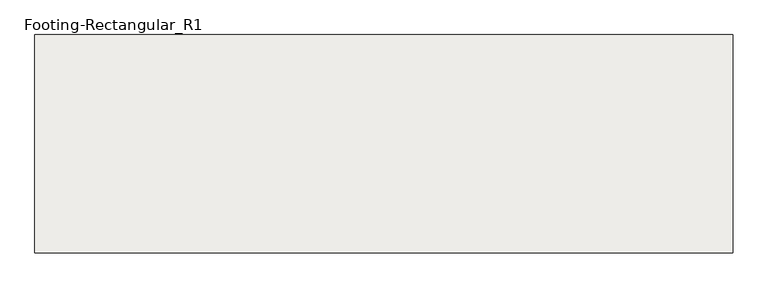
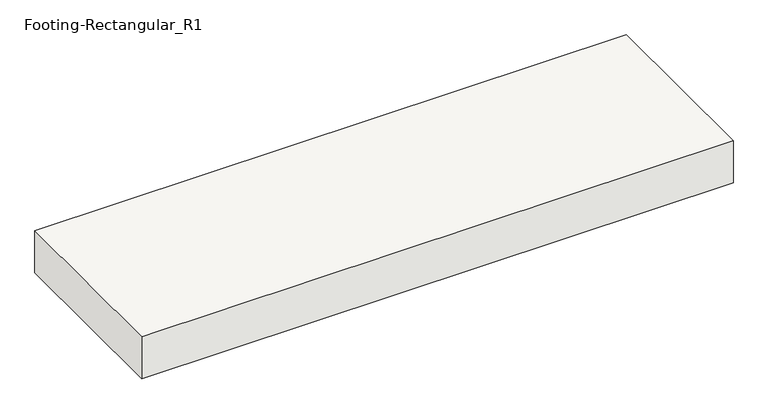
"""IFC4 building model written with IfcOpenShell, lengths in millimetres: slab geometry, Footing-Rectangular_R1 : H_SF_AR_S18_W8000xL2500xT500_Bitumen_F5."""

import ifcopenshell
import ifcopenshell.guid

model = None  # the IFC model being written
_history = None  # IfcOwnerHistory: only IFC2X3 demands one
_inside = {}  # id of a spatial element -> (the spatial element, [elements in it])
_under = {}  # id of a project, library or spatial element -> (it, [spatial elements below it])
_declared = {}  # id of a project -> (the project, [libraries it declares])
_typed = {}  # id of a type object -> (the type object, [elements of that type])
_made_of = {}  # id of a material, layer set ... -> (it, [elements and type objects made of it])


def new_model(schema):
    """Start an empty IFC model of exactly this schema.

    Asked for "IFC4X3", IfcOpenShell would pick the latest addendum, in which some entities
    have other attributes; the version numbers below select the first issue.
    IFC2X3 requires an IfcOwnerHistory on every rooted entity: one is made here for all.
    """
    global model, _history
    if schema == "IFC4X3":
        model = ifcopenshell.file(schema_version=(4, 3, 0, 0))
    else:
        model = ifcopenshell.file(schema=schema)
    _inside.clear()
    _under.clear()
    _declared.clear()
    _typed.clear()
    _made_of.clear()
    _history = None
    if model.schema == "IFC2X3":
        org = make("IfcOrganization", Name="unknown")
        user = make(
            "IfcPersonAndOrganization",
            ThePerson=make("IfcPerson", FamilyName="unknown"),
            TheOrganization=org,
        )
        app = make(
            "IfcApplication",
            ApplicationDeveloper=org,
            Version="unknown",
            ApplicationFullName="unknown",
            ApplicationIdentifier="unknown",
        )
        _history = make(
            "IfcOwnerHistory",
            OwningUser=user,
            OwningApplication=app,
            ChangeAction="ADDED",
            CreationDate=0,
        )
    return model


def make(cls, **values):
    """One entity of the class cls with the attributes given. An attribute that is None is left unset."""
    return model.create_entity(
        cls, **{name: value for name, value in values.items() if value is not None}
    )


def rooted(cls, **values):
    """An entity with a GlobalId (a new one), such as an element, a storey or a relation."""
    return make(cls, GlobalId=ifcopenshell.guid.new(), OwnerHistory=_history, **values)


def si_unit(unit_type, name, prefix=None):
    """IfcSIUnit, for example si_unit("LENGTHUNIT", "METRE", prefix="MILLI")."""
    return make("IfcSIUnit", UnitType=unit_type, Prefix=prefix, Name=name)


def assignment(units):
    """IfcUnitAssignment: the units of a project."""
    return None if units is None else make("IfcUnitAssignment", Units=units)


def point(xyz):
    """IfcCartesianPoint."""
    return None if xyz is None else make("IfcCartesianPoint", Coordinates=xyz)


def direction(xyz):
    """IfcDirection."""
    return None if xyz is None else make("IfcDirection", DirectionRatios=xyz)


def frame(location, z_axis=None, x_axis=None):
    """IfcAxis2Placement3D, a coordinate frame: its origin and axes. An axis left out is left unset."""
    return make(
        "IfcAxis2Placement3D",
        Location=point(location),
        Axis=direction(z_axis),
        RefDirection=direction(x_axis),
    )


def origin():
    """The frame at (0, 0, 0) with its axes left unset."""
    return frame((0.0, 0.0, 0.0))


def place(relative_to, where):
    """IfcLocalPlacement: puts the frame where relative to a parent placement (None: the world)."""
    return make(
        "IfcLocalPlacement", PlacementRelTo=relative_to, RelativePlacement=where
    )


def context(
    kind, dimensions, precision=None, world=None, true_north=None, identifier=None
):
    """IfcGeometricRepresentationContext, for example the 3D "Model" context."""
    return make(
        "IfcGeometricRepresentationContext",
        ContextIdentifier=identifier,
        ContextType=kind,
        CoordinateSpaceDimension=dimensions,
        Precision=precision,
        WorldCoordinateSystem=world,
        TrueNorth=true_north,
    )


def project(units=None, contexts=None):
    """IfcProject with its units and contexts."""
    return rooted(
        "IfcProject",
        Name="project",
        RepresentationContexts=contexts,
        UnitsInContext=assignment(units),
    )


def spatial(cls, under=None, at=None, **own):
    """A site, building, storey or space (cls), placed at a placement, below another one or the project."""
    s = rooted(cls, ObjectPlacement=at, **own)
    if under is not None:
        _under.setdefault(under.id(), (under, []))[1].append(s)
    return s


def polyline(points):
    """IfcPolyline through the points."""
    return make("IfcPolyline", Points=[point(p) for p in points])


def outline(outer, holes=None, kind="AREA"):
    """IfcArbitraryClosedProfileDef: a profile drawn as a closed curve; with holes, ...WithVoids."""
    if holes is None:
        return make("IfcArbitraryClosedProfileDef", ProfileType=kind, OuterCurve=outer)
    return make(
        "IfcArbitraryProfileDefWithVoids",
        ProfileType=kind,
        OuterCurve=outer,
        InnerCurves=holes,
    )


def extrude(swept, where, along, depth):
    """IfcExtrudedAreaSolid: the profile swept, set in the frame where, extruded along a direction by depth."""
    return make(
        "IfcExtrudedAreaSolid",
        SweptArea=swept,
        Position=where,
        ExtrudedDirection=direction(along),
        Depth=depth,
    )


def shape(context_of_items, identifier, shape_type, items):
    """IfcShapeRepresentation: the items that make up one representation, for example the "Body"."""
    return make(
        "IfcShapeRepresentation",
        ContextOfItems=context_of_items,
        RepresentationIdentifier=identifier,
        RepresentationType=shape_type,
        Items=items,
    )


def source(mapping_origin, context_of_items, identifier, shape_type, items):
    """IfcRepresentationMap: a shape defined once, which mapped items show again and again."""
    return make(
        "IfcRepresentationMap",
        MappingOrigin=mapping_origin,
        MappedRepresentation=shape(context_of_items, identifier, shape_type, items),
    )


def transform(
    local_origin,
    x_axis=None,
    y_axis=None,
    z_axis=None,
    scale=None,
    scale2=None,
    scale3=None,
    uniform=True,
):
    """IfcCartesianTransformationOperator3D, or its non-uniform kind. x_axis, y_axis, z_axis: its Axis1, 2, 3."""
    if uniform:
        return make(
            "IfcCartesianTransformationOperator3D",
            Axis1=direction(x_axis),
            Axis2=direction(y_axis),
            LocalOrigin=point(local_origin),
            Scale=scale,
            Axis3=direction(z_axis),
        )
    return make(
        "IfcCartesianTransformationOperator3DnonUniform",
        Axis1=direction(x_axis),
        Axis2=direction(y_axis),
        LocalOrigin=point(local_origin),
        Scale=scale,
        Axis3=direction(z_axis),
        Scale2=scale2,
        Scale3=scale3,
    )


def mapped(mapping_source, mapping_target):
    """IfcMappedItem: shows the shape of a source again, moved by a transform."""
    return make(
        "IfcMappedItem", MappingSource=mapping_source, MappingTarget=mapping_target
    )


def made_of(thing, what):
    """Note that an element or type object is made of a material, layer set ...; save() writes the relation."""
    if what is not None:
        _made_of.setdefault(what.id(), (what, []))[1].append(thing)
    return thing


def element(
    cls,
    number,
    at=None,
    inside=None,
    cuts=None,
    type_object=None,
    material=None,
    context=None,
    identifier="Body",
    shape_type=None,
    held_by="IfcProductDefinitionShape",
    body=None,
    shapes=None,
    **own,
):
    """One element of the class cls, such as IfcWall. Its Tag is "e" and its number.

    at: its placement. inside: the storey or other place that contains it. cuts: it is an
    opening in that element (IfcRelVoidsElement). A single representation is given by context,
    identifier, shape_type and body (its items); several are given by shapes. held_by: the class
    of the entity that holds the representations. save() writes the other relations.
    """
    e = rooted(cls, Tag="e%d" % number, ObjectPlacement=at, **own)
    if body is not None:
        shapes = [shape(context, identifier, shape_type, body)]
    if shapes is not None:
        e.Representation = make(held_by, Representations=shapes)
    if inside is not None:
        _inside.setdefault(inside.id(), (inside, []))[1].append(e)
    if cuts is not None:
        rooted(
            "IfcRelVoidsElement", RelatingBuildingElement=cuts, RelatedOpeningElement=e
        )
    if type_object is not None:
        _typed.setdefault(type_object.id(), (type_object, []))[1].append(e)
    return made_of(e, material)


def aggregate(whole, parts):
    """IfcRelAggregates: a whole, such as a stair, and the parts it consists of."""
    return rooted("IfcRelAggregates", RelatingObject=whole, RelatedObjects=parts)


def save(model, path):
    """Write the relations noted so far, then the file.

    IfcRelAggregates (storeys below a building ...), IfcRelContainedInSpatialStructure (elements
    in a storey), IfcRelDefinesByType, IfcRelAssociatesMaterial and IfcRelDeclares: one each for
    every whole, place, type object, material and project.
    """
    for whole, parts in _under.values():
        aggregate(whole, parts)
    for where, things in _inside.values():
        rooted(
            "IfcRelContainedInSpatialStructure",
            RelatedElements=things,
            RelatingStructure=where,
        )
    for kind, things in _typed.values():
        rooted("IfcRelDefinesByType", RelatedObjects=things, RelatingType=kind)
    for what, things in _made_of.values():
        rooted("IfcRelAssociatesMaterial", RelatedObjects=things, RelatingMaterial=what)
    for by, libraries in _declared.values():
        rooted("IfcRelDeclares", RelatingContext=by, RelatedDefinitions=libraries)
    model.write(path)


def footing_rectangular_r1_282b4f06(model_context):
    return source(origin(), model_context, "Body", "SweptSolid", [
        extrude(outline(polyline([(4000.0, 1250.0), (4000.0, -1250.0), (-4000.0, -1250.0), (-4000.0, 1250.0), (4000.0, 1250.0)])), frame((0.0, 0.0, -600.0), z_axis=(0.0, 0.0, 1.0), x_axis=(1.0, 0.0, 0.0)), (0.0, 0.0, 1.0), 600.0),
    ])


if __name__ == "__main__":
    model = new_model("IFC4")
    model_context = context("Model", 3, world=origin())
    ifc_project = project(units=[si_unit("LENGTHUNIT", "METRE", prefix="MILLI")], contexts=[model_context])
    site = spatial("IfcSite", under=ifc_project)
    building = spatial("IfcBuilding", under=site)
    placement = place(None, origin())
    footing_rectangular_r1_shape = footing_rectangular_r1_282b4f06(model_context)
    element("IfcSlab", 1, ObjectType="Footing-Rectangular_R1 : H_SF_AR_S18_W8000xL2500xT500_Bitumen_F5", at=placement, inside=building, context=model_context, shape_type="MappedRepresentation", body=[
        mapped(footing_rectangular_r1_shape, transform((0.0, 0.0, 0.0), x_axis=(1.0, 0.0, 0.0), y_axis=(0.0, 1.0, 0.0), z_axis=(0.0, 0.0, 1.0))),
    ])
    save(model, "model.ifc")

# Revit data of these elements
# Type "Footing-Rectangular_R1 : H_SF_AR_S18_W8000xL2500xT500_Bitumen_F5"
#   Type Mark = "F5"
#   Top bar = "D25@300"
#   Description = "UG Shallow Foundation"
#   Bottom bar = "D20@300"
#   Width = 8000 mm
#   Length = 2500 mm
#   Foundation Thickness = 600 mm
#   Structural Material [instance default] = none
#   Assembly Code = ""
